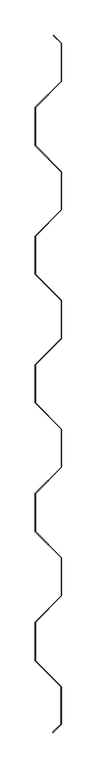
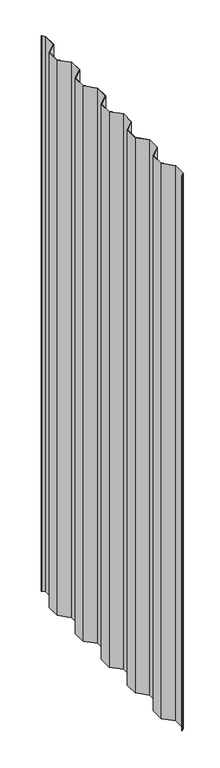
"""IFC4 building model written with IfcOpenShell, lengths in millimetres: proxy geometry, MBCI 7.2-V Panel37 : MBCI 7.2-V Panel-1."""

from ifc_helpers import new_model, si_unit, frame, origin, place, context, project, spatial, polyline, outline, extrude, source, transform, mapped, element, save


def generic_models_8da91ac8(model_context):
    return source(origin(), model_context, "Body", "SweptSolid", [
        extrude(outline(polyline([(587368.2461489, -533059.7470706), (587330.7557489, -533097.2374706), (587330.7557489, -533151.0249614), (587368.2461489, -533188.5153614), (587368.2461489, -533242.6270706), (587330.7557489, -533280.1174706), (587330.7557489, -533333.9049614), (587368.2461489, -533371.3953614), (587368.2461489, -533425.5070706), (587330.7557489, -533462.9974706), (587330.7557489, -533516.7849614), (587368.2461489, -533554.2753614), (587368.2461489, -533608.3870706), (587330.7557489, -533645.8774706), (587330.7557489, -533699.6649614), (587368.2461489, -533737.1553614), (587368.2461489, -533791.2670706), (587330.7557489, -533828.7574706), (587330.7557489, -533883.4085614), (587367.6365489, -533920.2893614), (587367.6365489, -533973.8706614), (587355.9658262, -533985.5413841), (587355.9108025, -533984.7545088), (587367.0412364, -533973.6240749), (587367.0412364, -533920.5359479), (587330.1604364, -533883.6551479), (587330.1604364, -533828.510884), (587367.6508364, -533791.020484), (587367.6508364, -533737.4019479), (587330.1604364, -533699.9115479), (587330.1604364, -533645.630884), (587367.6508364, -533608.140484), (587367.6508364, -533554.5219479), (587330.1604364, -533517.0315479), (587330.1604364, -533462.750884), (587367.6508364, -533425.260484), (587367.6508364, -533371.6419479), (587330.1604364, -533334.1515479), (587330.1604364, -533279.870884), (587367.6508364, -533242.380484), (587367.6508364, -533188.7619479), (587330.1604364, -533151.2715479), (587330.1604364, -533096.990884), (587367.6508364, -533059.500484), (587367.6508364, -533005.8819479), (587356.8035899, -532995.0347014), (587356.8455148, -532994.2347273), (587368.2461489, -533005.6353614), (587368.2461489, -533059.7470706)])), frame((0.0, 0.0, 51.59375), z_axis=(0.0, 0.0, 1.0), x_axis=(1.0, 0.0, 0.0)), (0.0, 0.0, 1.0), 2386.80625),
    ])


if __name__ == "__main__":
    model = new_model("IFC4")
    model_context = context("Model", 3, world=origin())
    ifc_project = project(units=[si_unit("LENGTHUNIT", "METRE", prefix="MILLI")], contexts=[model_context])
    site = spatial("IfcSite", under=ifc_project)
    building = spatial("IfcBuilding", under=site)
    placement = place(None, origin())
    generic_models_shape = generic_models_8da91ac8(model_context)
    element("IfcBuildingElementProxy", 1, Name="MBCI 7.2-V Panel37 : MBCI 7.2-V Panel-1", ObjectType="MBCI 7.2-V Panel37 : MBCI 7.2-V Panel-1", at=placement, inside=building, context=model_context, shape_type="MappedRepresentation", body=[
        mapped(generic_models_shape, transform((0.0, 0.0, 0.0), x_axis=(1.0, 0.0, 0.0), y_axis=(0.0, 1.0, 0.0), z_axis=(0.0, 0.0, 1.0))),
    ])
    save(model, "model.ifc")

# Revit data of these elements
# Element 1 (IfcBuildingElementProxy, "MBCI 7.2-V Panel37 : MBCI 7.2-V Panel-1")
#   Materials on its faces: "MTL PANEL"
# Materials
#   "MTL PANEL": class "Generic", colour RGB 239 242 240, transparency 0, Cost = 0
